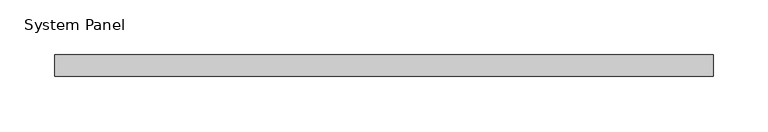
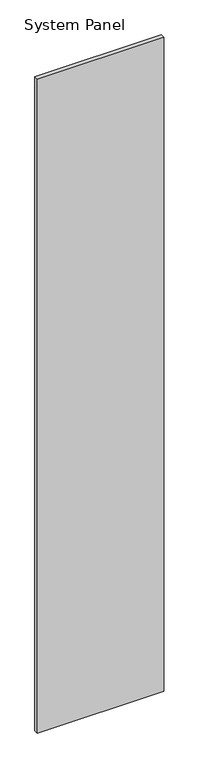
"""IFC4 building model written with IfcOpenShell, lengths in millimetres: plate geometry, System Panel : WWm-Glass-20mm-10mmOffset."""

from ifc_helpers import new_model, si_unit, origin, origin_with_axes, place, context, project, spatial, polyline, outline, extrude, source, transform, mapped, element, save


def system_panel_f4aabc45(model_context):
    return source(origin(), model_context, "Body", "SweptSolid", [
        extrude(outline(polyline([(302.0, 0.0), (-302.0, 0.0), (-302.0, 20.0), (302.0, 20.0), (302.0, 0.0)])), origin_with_axes(), (0.0, 0.0, 1.0), 3300.0),
    ])


if __name__ == "__main__":
    model = new_model("IFC4")
    model_context = context("Model", 3, world=origin())
    ifc_project = project(units=[si_unit("LENGTHUNIT", "METRE", prefix="MILLI")], contexts=[model_context])
    site = spatial("IfcSite", under=ifc_project)
    building = spatial("IfcBuilding", under=site)
    placement = place(None, origin())
    system_panel_shape = system_panel_f4aabc45(model_context)
    element("IfcPlate", 1, ObjectType="System Panel : WWm-Glass-20mm-10mmOffset", at=placement, inside=building, context=model_context, shape_type="MappedRepresentation", body=[
        mapped(system_panel_shape, transform((0.0, 0.0, 0.0), x_axis=(1.0, 0.0, 0.0), y_axis=(0.0, 1.0, 0.0), z_axis=(0.0, 0.0, 1.0))),
    ])
    save(model, "model.ifc")

# Revit data of these elements
# Type "System Panel : WWm-Glass-20mm-10mmOffset"
#   Finish = ""
# Element 1 (IfcPlate, "System Panel : WWm-Glass-20mm-10mmOffset")
#   Materials on its faces: "WW-EC-GL-Storefront"
# Materials
#   "WW-EC-GL-Storefront": class "Glass", colour RGB 236 240 239, transparency 0.85, Description = "Storefront Glass", Cost = 0
